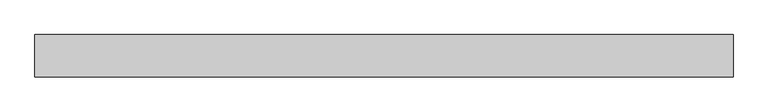
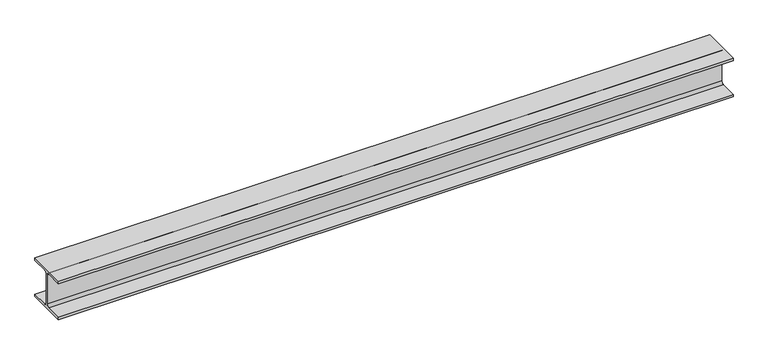
"""IFC4 building model written with IfcOpenShell, lengths in millimetres: beam geometry, 0912_Steel Framing_H-KSD3502 : H_SB_ASB_H-200x200x8x12."""

from ifc_helpers import new_model, si_unit, point, frame, frame_2d, origin, place, context, project, spatial, polyline, circle_curve, trimmed, segment, composite_curve, outline, extrude, source, transform, mapped, element, save


def beam_c4df9c99(model_context):
    return source(origin(), model_context, "Body", "SweptSolid", [
        extrude(outline(composite_curve([segment(polyline([(100.0, -88.0), (100.0, -100.0), (-100.0, -100.0), (-100.0, -88.0), (-17.0, -88.0)]), True, "CONTINUOUS"), segment(trimmed(circle_curve(frame_2d((-17.0, -75.0)), 13.0), [point((-17.0, -88.0))], [point((-4.0, -75.0))], True, "CARTESIAN"), True, "CONTINUOUS"), segment(polyline([(-4.0, -75.0), (-4.0, 75.0)]), True, "CONTINUOUS"), segment(trimmed(circle_curve(frame_2d((-17.0, 75.0)), 13.0), [point((-4.0, 75.0))], [point((-17.0, 88.0))], True, "CARTESIAN"), True, "CONTINUOUS"), segment(polyline([(-17.0, 88.0), (-100.0, 88.0), (-100.0, 100.0), (100.0, 100.0), (100.0, 88.0), (17.0, 88.0)]), True, "CONTINUOUS"), segment(trimmed(circle_curve(frame_2d((17.0, 75.0)), 13.0), [point((17.0, 88.0))], [point((4.0, 75.0))], True, "CARTESIAN"), True, "CONTINUOUS"), segment(polyline([(4.0, 75.0), (4.0, -75.0)]), True, "CONTINUOUS"), segment(trimmed(circle_curve(frame_2d((17.0, -75.0)), 13.0), [point((4.0, -75.0))], [point((17.0, -88.0))], True, "CARTESIAN"), True, "CONTINUOUS"), segment(polyline([(17.0, -88.0), (100.0, -88.0)]), True, "CONTINUOUS")], self_intersect=False)), frame((-1611.7677924, 0.0, 0.0), z_axis=(1.0, 0.0, 0.0), x_axis=(0.0, 1.0, 0.0)), (0.0, 0.0, 1.0), 3310.7044425),
    ])


if __name__ == "__main__":
    model = new_model("IFC4")
    model_context = context("Model", 3, world=origin())
    ifc_project = project(units=[si_unit("LENGTHUNIT", "METRE", prefix="MILLI")], contexts=[model_context])
    site = spatial("IfcSite", under=ifc_project)
    building = spatial("IfcBuilding", under=site)
    placement = place(None, origin())
    beam_shape = beam_c4df9c99(model_context)
    element("IfcBeam", 1, ObjectType="0912_Steel Framing_H-KSD3502 : H_SB_ASB_H-200x200x8x12", at=placement, inside=building, context=model_context, shape_type="MappedRepresentation", body=[
        mapped(beam_shape, transform((0.0, 0.0, 0.0), x_axis=(1.0, 0.0, 0.0), y_axis=(0.0, 1.0, 0.0), z_axis=(0.0, 0.0, 1.0))),
    ])
    save(model, "model.ifc")

# Revit data of these elements
# Type "0912_Steel Framing_H-KSD3502 : H_SB_ASB_H-200x200x8x12"
#   H_WM Code_1 = "S01AA002-00001 | Main Steel Structure Fabrication Work | Shelter/Building | Medium Steel - Standard (90KG/M>Weight≥30KG/M) | Material: (   )"
#   H_WM Code_2 = "S03AA028-00001 | Main Steel Structure Erection Work | Shelter/Building | Medium Steel (90KG/M>Weight≥30KG/M) | Material: (   )"
#   H_WM Code_3 = "S01AA010-00001 | Main Steel Structure Fabrication Work | Shelter/Building | Steel Painting/Coating | for Non-Fireproofed Steel Surface, Surface Preparation, Primer, Second & Final Coat | Material: (   )"
#   H_Q'ty Cal Type Tag = "SB-Q2"
#   Width = 20.0 cm
#   Web Thickness = 0.8 cm
#   Web Fillet = 1.3 cm
#   Warping Constant = 141000.0 cm⁶
#   W = 0
#   Torsional Moment of Inertia = 26.2485 cm⁴
#   Section Area = 63.53 cm²
#   Plastic Modulus weak axis = 244.0 cm³
#   Plastic Modulus strong axis = 525.0 cm³
#   Perimeter = 1.16 m²/m
#   Nominal Weight = 49.90 kgf/m
#   Moment of Inertia weak axis = 1600.00 cm⁴
#   Moment of Inertia strong axis = 4720.00 cm⁴
#   Height = 20.0 cm
#   Flange Thickness = 1.2 cm
#   Elastic Modulus weak axis = 160.0 cm³
#   Elastic Modulus strong axis = 472.0 cm³
#   Centroid Vertical = 10.0 cm
#   Centroid Horizontal = 10.0 cm
#   Ix = 47200000
#   Length [instance default] = 1.5240 m
#   Zx = 525000
#   b = 0.2000 m
#   h = 0.2000 m
#   r = 0.0130 m
#   s = 0.0080 m
#   t = 0.0120 m
#   A = 0.006353 m²
#   Structural Material [instance default] = Steel, 45-345
#   Assembly Code = ""
# Element 1 (IfcBeam, "0912_Steel Framing_H-KSD3502 : H_SB_ASB_H-200x200x8x12")
#   Structural Material = none
# Materials
#   "Steel, 45-345": class "Metal", colour RGB 189 187 185, transparency 0, Description = "Steel 345 MPa", Cost = 0
